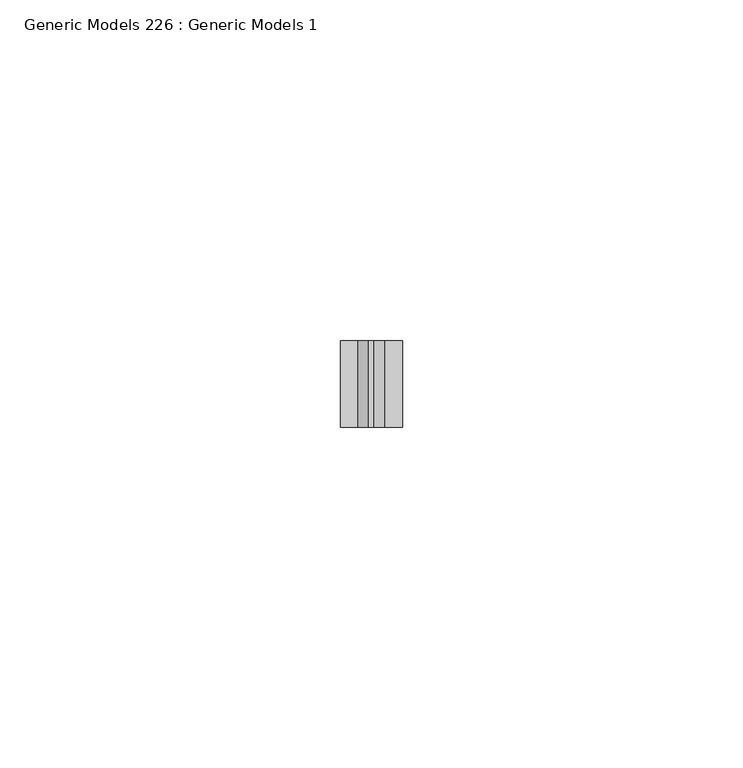
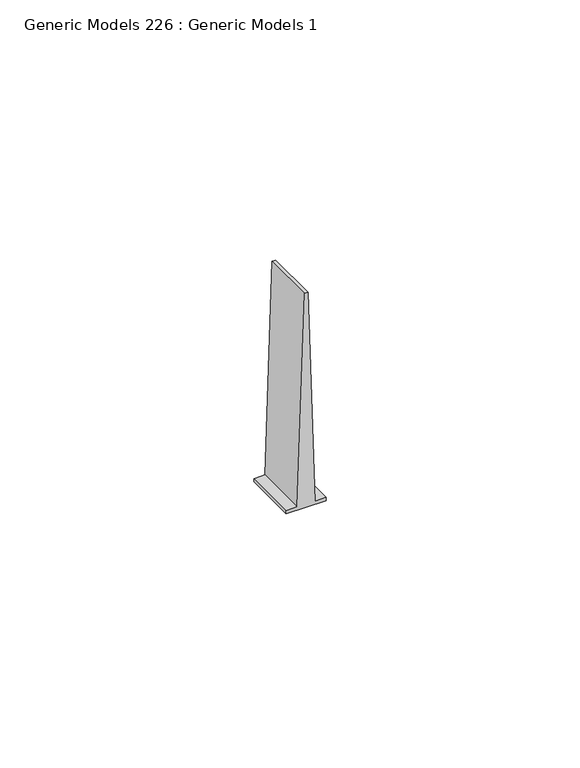
"""IFC4 building model written with IfcOpenShell, lengths in millimetres: proxy geometry, Generic Models 226 : Generic Models 1."""

import ifcopenshell
import ifcopenshell.guid

model = None  # the IFC model being written
_history = None  # IfcOwnerHistory: only IFC2X3 demands one
_inside = {}  # id of a spatial element -> (the spatial element, [elements in it])
_under = {}  # id of a project, library or spatial element -> (it, [spatial elements below it])
_declared = {}  # id of a project -> (the project, [libraries it declares])
_typed = {}  # id of a type object -> (the type object, [elements of that type])
_made_of = {}  # id of a material, layer set ... -> (it, [elements and type objects made of it])


def new_model(schema):
    """Start an empty IFC model of exactly this schema.

    Asked for "IFC4X3", IfcOpenShell would pick the latest addendum, in which some entities
    have other attributes; the version numbers below select the first issue.
    IFC2X3 requires an IfcOwnerHistory on every rooted entity: one is made here for all.
    """
    global model, _history
    if schema == "IFC4X3":
        model = ifcopenshell.file(schema_version=(4, 3, 0, 0))
    else:
        model = ifcopenshell.file(schema=schema)
    _inside.clear()
    _under.clear()
    _declared.clear()
    _typed.clear()
    _made_of.clear()
    _history = None
    if model.schema == "IFC2X3":
        org = make("IfcOrganization", Name="unknown")
        user = make(
            "IfcPersonAndOrganization",
            ThePerson=make("IfcPerson", FamilyName="unknown"),
            TheOrganization=org,
        )
        app = make(
            "IfcApplication",
            ApplicationDeveloper=org,
            Version="unknown",
            ApplicationFullName="unknown",
            ApplicationIdentifier="unknown",
        )
        _history = make(
            "IfcOwnerHistory",
            OwningUser=user,
            OwningApplication=app,
            ChangeAction="ADDED",
            CreationDate=0,
        )
    return model


def make(cls, **values):
    """One entity of the class cls with the attributes given. An attribute that is None is left unset."""
    return model.create_entity(
        cls, **{name: value for name, value in values.items() if value is not None}
    )


def rooted(cls, **values):
    """An entity with a GlobalId (a new one), such as an element, a storey or a relation."""
    return make(cls, GlobalId=ifcopenshell.guid.new(), OwnerHistory=_history, **values)


def si_unit(unit_type, name, prefix=None):
    """IfcSIUnit, for example si_unit("LENGTHUNIT", "METRE", prefix="MILLI")."""
    return make("IfcSIUnit", UnitType=unit_type, Prefix=prefix, Name=name)


def assignment(units):
    """IfcUnitAssignment: the units of a project."""
    return None if units is None else make("IfcUnitAssignment", Units=units)


def point(xyz):
    """IfcCartesianPoint."""
    return None if xyz is None else make("IfcCartesianPoint", Coordinates=xyz)


def direction(xyz):
    """IfcDirection."""
    return None if xyz is None else make("IfcDirection", DirectionRatios=xyz)


def frame(location, z_axis=None, x_axis=None):
    """IfcAxis2Placement3D, a coordinate frame: its origin and axes. An axis left out is left unset."""
    return make(
        "IfcAxis2Placement3D",
        Location=point(location),
        Axis=direction(z_axis),
        RefDirection=direction(x_axis),
    )


def origin():
    """The frame at (0, 0, 0) with its axes left unset."""
    return frame((0.0, 0.0, 0.0))


def place(relative_to, where):
    """IfcLocalPlacement: puts the frame where relative to a parent placement (None: the world)."""
    return make(
        "IfcLocalPlacement", PlacementRelTo=relative_to, RelativePlacement=where
    )


def context(
    kind, dimensions, precision=None, world=None, true_north=None, identifier=None
):
    """IfcGeometricRepresentationContext, for example the 3D "Model" context."""
    return make(
        "IfcGeometricRepresentationContext",
        ContextIdentifier=identifier,
        ContextType=kind,
        CoordinateSpaceDimension=dimensions,
        Precision=precision,
        WorldCoordinateSystem=world,
        TrueNorth=true_north,
    )


def project(units=None, contexts=None):
    """IfcProject with its units and contexts."""
    return rooted(
        "IfcProject",
        Name="project",
        RepresentationContexts=contexts,
        UnitsInContext=assignment(units),
    )


def spatial(cls, under=None, at=None, **own):
    """A site, building, storey or space (cls), placed at a placement, below another one or the project."""
    s = rooted(cls, ObjectPlacement=at, **own)
    if under is not None:
        _under.setdefault(under.id(), (under, []))[1].append(s)
    return s


def polyline(points):
    """IfcPolyline through the points."""
    return make("IfcPolyline", Points=[point(p) for p in points])


def outline(outer, holes=None, kind="AREA"):
    """IfcArbitraryClosedProfileDef: a profile drawn as a closed curve; with holes, ...WithVoids."""
    if holes is None:
        return make("IfcArbitraryClosedProfileDef", ProfileType=kind, OuterCurve=outer)
    return make(
        "IfcArbitraryProfileDefWithVoids",
        ProfileType=kind,
        OuterCurve=outer,
        InnerCurves=holes,
    )


def extrude(swept, where, along, depth):
    """IfcExtrudedAreaSolid: the profile swept, set in the frame where, extruded along a direction by depth."""
    return make(
        "IfcExtrudedAreaSolid",
        SweptArea=swept,
        Position=where,
        ExtrudedDirection=direction(along),
        Depth=depth,
    )


def shape(context_of_items, identifier, shape_type, items):
    """IfcShapeRepresentation: the items that make up one representation, for example the "Body"."""
    return make(
        "IfcShapeRepresentation",
        ContextOfItems=context_of_items,
        RepresentationIdentifier=identifier,
        RepresentationType=shape_type,
        Items=items,
    )


def source(mapping_origin, context_of_items, identifier, shape_type, items):
    """IfcRepresentationMap: a shape defined once, which mapped items show again and again."""
    return make(
        "IfcRepresentationMap",
        MappingOrigin=mapping_origin,
        MappedRepresentation=shape(context_of_items, identifier, shape_type, items),
    )


def transform(
    local_origin,
    x_axis=None,
    y_axis=None,
    z_axis=None,
    scale=None,
    scale2=None,
    scale3=None,
    uniform=True,
):
    """IfcCartesianTransformationOperator3D, or its non-uniform kind. x_axis, y_axis, z_axis: its Axis1, 2, 3."""
    if uniform:
        return make(
            "IfcCartesianTransformationOperator3D",
            Axis1=direction(x_axis),
            Axis2=direction(y_axis),
            LocalOrigin=point(local_origin),
            Scale=scale,
            Axis3=direction(z_axis),
        )
    return make(
        "IfcCartesianTransformationOperator3DnonUniform",
        Axis1=direction(x_axis),
        Axis2=direction(y_axis),
        LocalOrigin=point(local_origin),
        Scale=scale,
        Axis3=direction(z_axis),
        Scale2=scale2,
        Scale3=scale3,
    )


def mapped(mapping_source, mapping_target):
    """IfcMappedItem: shows the shape of a source again, moved by a transform."""
    return make(
        "IfcMappedItem", MappingSource=mapping_source, MappingTarget=mapping_target
    )


def made_of(thing, what):
    """Note that an element or type object is made of a material, layer set ...; save() writes the relation."""
    if what is not None:
        _made_of.setdefault(what.id(), (what, []))[1].append(thing)
    return thing


def element(
    cls,
    number,
    at=None,
    inside=None,
    cuts=None,
    type_object=None,
    material=None,
    context=None,
    identifier="Body",
    shape_type=None,
    held_by="IfcProductDefinitionShape",
    body=None,
    shapes=None,
    **own,
):
    """One element of the class cls, such as IfcWall. Its Tag is "e" and its number.

    at: its placement. inside: the storey or other place that contains it. cuts: it is an
    opening in that element (IfcRelVoidsElement). A single representation is given by context,
    identifier, shape_type and body (its items); several are given by shapes. held_by: the class
    of the entity that holds the representations. save() writes the other relations.
    """
    e = rooted(cls, Tag="e%d" % number, ObjectPlacement=at, **own)
    if body is not None:
        shapes = [shape(context, identifier, shape_type, body)]
    if shapes is not None:
        e.Representation = make(held_by, Representations=shapes)
    if inside is not None:
        _inside.setdefault(inside.id(), (inside, []))[1].append(e)
    if cuts is not None:
        rooted(
            "IfcRelVoidsElement", RelatingBuildingElement=cuts, RelatedOpeningElement=e
        )
    if type_object is not None:
        _typed.setdefault(type_object.id(), (type_object, []))[1].append(e)
    return made_of(e, material)


def aggregate(whole, parts):
    """IfcRelAggregates: a whole, such as a stair, and the parts it consists of."""
    return rooted("IfcRelAggregates", RelatingObject=whole, RelatedObjects=parts)


def save(model, path):
    """Write the relations noted so far, then the file.

    IfcRelAggregates (storeys below a building ...), IfcRelContainedInSpatialStructure (elements
    in a storey), IfcRelDefinesByType, IfcRelAssociatesMaterial and IfcRelDeclares: one each for
    every whole, place, type object, material and project.
    """
    for whole, parts in _under.values():
        aggregate(whole, parts)
    for where, things in _inside.values():
        rooted(
            "IfcRelContainedInSpatialStructure",
            RelatedElements=things,
            RelatingStructure=where,
        )
    for kind, things in _typed.values():
        rooted("IfcRelDefinesByType", RelatedObjects=things, RelatingType=kind)
    for what, things in _made_of.values():
        rooted("IfcRelAssociatesMaterial", RelatedObjects=things, RelatingMaterial=what)
    for by, libraries in _declared.values():
        rooted("IfcRelDeclares", RelatingContext=by, RelatedDefinitions=libraries)
    model.write(path)


def generic_models_226_generic_models_1_7dc37832(model_context):
    return source(origin(), model_context, "Body", "SweptSolid", [
        extrude(outline(polyline([(5263.35625, 49733.4159), (5263.35625, 49742.5091), (5264.15, 49742.5091), (5264.15, 49739.9592364), (5314.95, 49738.3618473), (5314.95, 49737.5631527), (5264.15, 49735.9657636), (5264.15, 49733.4159), (5263.35625, 49733.4159)])), frame((0.0, 565.15, 0.0), z_axis=(0.0, 1.0, 0.0), x_axis=(0.0, 0.0, 1.0)), (0.0, 0.0, 1.0), 12.7),
    ])


if __name__ == "__main__":
    model = new_model("IFC4")
    model_context = context("Model", 3, world=origin())
    ifc_project = project(units=[si_unit("LENGTHUNIT", "METRE", prefix="MILLI")], contexts=[model_context])
    site = spatial("IfcSite", under=ifc_project)
    building = spatial("IfcBuilding", under=site)
    placement = place(None, origin())
    generic_models_226_generic_models_1_shape = generic_models_226_generic_models_1_7dc37832(model_context)
    element("IfcBuildingElementProxy", 1, Name="Generic Models 226 : Generic Models 1", ObjectType="Generic Models 226 : Generic Models 1", at=placement, inside=building, context=model_context, shape_type="MappedRepresentation", body=[
        mapped(generic_models_226_generic_models_1_shape, transform((0.0, 0.0, 0.0), x_axis=(1.0, 0.0, 0.0), y_axis=(0.0, 1.0, 0.0), z_axis=(0.0, 0.0, 1.0))),
    ])
    save(model, "model.ifc")

# Revit data of these elements
# Element 1 (IfcBuildingElementProxy, "Generic Models 226 : Generic Models 1")
#   Materials on its faces: "METAL RUNNER CHANNEL; FASTEN @ 24\" O.C."
# Materials
#   "METAL RUNNER CHANNEL; FASTEN @ 24\" O.C.": class "Unassigned", colour RGB 210 209 208, transparency 0, Keynote = "M05121300.02", Cost = 0
